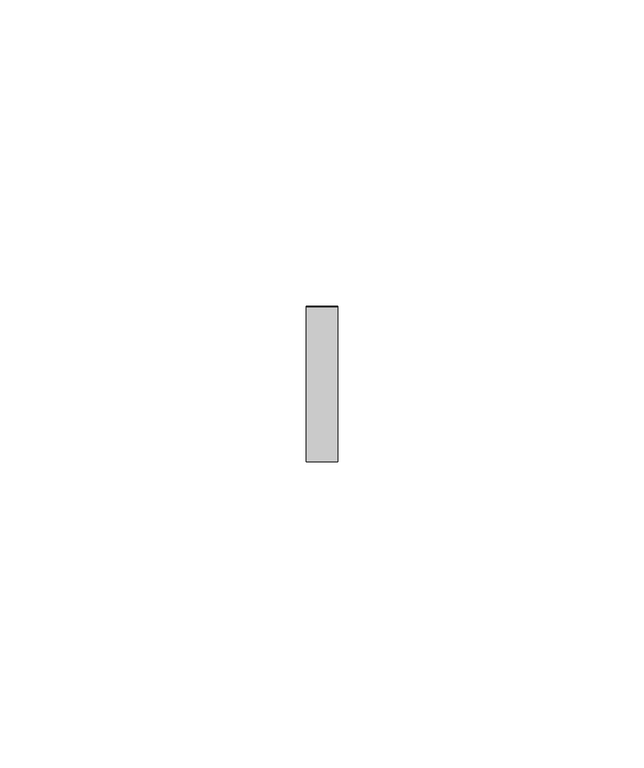
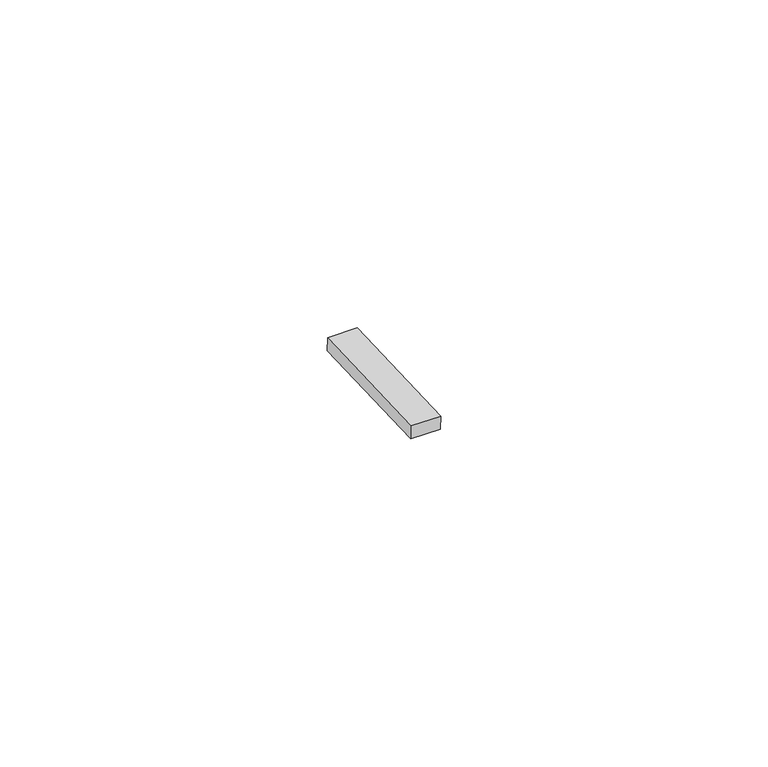
"""IFC4 building model written with IfcOpenShell, lengths in millimetres: proxy geometry, Inner panel:Inner panel:1:Inner panel:1 : Inner panel:Inner panel:300324:2:Inner panel:1:Inner panel:1 : Inner panel:Inner panel:300324:2 : Inner panel:Inner panel:1:Inner panel:1 : Inner panel:Inner panel:300324:300043:107 : Inner panel:Inner panel:1:Inner panel:1 : Inner panel:Inner panel:300324:2:Inner panel:1:Inner panel:1 : Inner panel:Inner panel:300324:2 : Inner panel:Inner panel:1:Inner panel:1 : Inner panel:Inner panel:300324:300043:308120."""

from ifc_helpers import new_model, si_unit, frame, origin, place, context, project, spatial, polyline, outline, extrude, source, transform, mapped, element, save


def generic_models_22f333e8(model_context):
    return source(origin(), model_context, "Body", "SweptSolid", [
        extrude(outline(polyline([(0.0, -25.3999999), (0.0, 0.0), (5.2138089, 0.0), (5.2138089, -25.3999999), (0.0, -25.3999999)])), frame((593530.195117, -577413.7950993, 4016.01903), z_axis=(0.0, -0.041630544712223896, 0.9991330730923502), x_axis=(-1.0, 0.0, 0.0)), (0.0, 0.0, 1.0), 2.4763745),
    ])


if __name__ == "__main__":
    model = new_model("IFC4")
    model_context = context("Model", 3, world=origin())
    ifc_project = project(units=[si_unit("LENGTHUNIT", "METRE", prefix="MILLI")], contexts=[model_context])
    site = spatial("IfcSite", under=ifc_project)
    building = spatial("IfcBuilding", under=site)
    placement = place(None, origin())
    generic_models_shape = generic_models_22f333e8(model_context)
    element("IfcBuildingElementProxy", 1, Name="Inner panel:Inner panel:1:Inner panel:1 : Inner panel:Inner panel:300324:2:Inner panel:1:Inner panel:1 : Inner panel:Inner panel:300324:2 : Inner panel:Inner panel:1:Inner panel:1 : Inner panel:Inner panel:300324:300043:107 : Inner panel:Inner panel:1:Inner panel:1 : Inner panel:Inner panel:300324:2:Inner panel:1:Inner panel:1 : Inner panel:Inner panel:300324:2 : Inner panel:Inner panel:1:Inner panel:1 : Inner panel:Inner panel:300324:300043:308120", ObjectType="Inner panel:Inner panel:1:Inner panel:1 : Inner panel:Inner panel:300324:2:Inner panel:1:Inner panel:1 : Inner panel:Inner panel:300324:2 : Inner panel:Inner panel:1:Inner panel:1 : Inner panel:Inner panel:300324:300043:107 : Inner panel:Inner panel:1:Inner panel:1 : Inner panel:Inner panel:300324:2:Inner panel:1:Inner panel:1 : Inner panel:Inner panel:300324:2 : Inner panel:Inner panel:1:Inner panel:1 : Inner panel:Inner panel:300324:300043:308120", at=placement, inside=building, context=model_context, shape_type="MappedRepresentation", body=[
        mapped(generic_models_shape, transform((0.0, 0.0, 0.0), x_axis=(1.0, 0.0, 0.0), y_axis=(0.0, 1.0, 0.0), z_axis=(0.0, 0.0, 1.0))),
    ])
    save(model, "model.ifc")

# Revit data of these elements
# Type "Inner panel:Inner panel:1:Inner panel:1 : Inner panel:Inner panel:300324:2:Inner panel:1:Inner panel:1 : Inner panel:Inner panel:300324:2 : Inner panel:Inner panel:1:Inner panel:1 : Inner panel:Inner panel:300324:300043:107 : Inner panel:Inner panel:1:Inner panel:1 : Inner panel:Inner panel:300324:2:Inner panel:1:Inner panel:1 : Inner panel:Inner panel:300324:2 : Inner panel:Inner panel:1:Inner panel:1 : Inner panel:Inner panel:300324:300043:308120"
#   NameOverride = "Inner panel:Inner panel:1:Inner panel:1 : Inner panel:Inner panel:300324:2:Inner panel:1:Inner panel:1 : Inner panel:Inner panel:300324:2 : Inner panel:Inner panel:1:Inner panel:1 : Inner panel:Inner panel:300324:300043:308120"
#   ObjectTypeOverride = "Inner panel:1:Inner panel:1 : Inner panel:Inner panel:300324:2 : Inner panel:Inner panel:1:Inner panel:1 : Inner panel:Inner panel:300324:300043"
#   Reference = "Inner panel"
#   Tag = "308120"
# Element 1 (IfcBuildingElementProxy, "Inner panel:Inner panel:1:Inner panel:1 : Inner panel:Inner panel:300324:2:Inner panel:1:Inner panel:1 : Inner panel:Inner panel:300324:2 : Inner panel:Inner panel:1:Inner panel:1 : Inner panel:Inner panel:300324:300043:107 : Inner panel:Inner panel:1:Inner panel:1 : Inner panel:Inner panel:300324:2:Inner panel:1:Inner panel:1 : Inner panel:Inner panel:300324:2 : Inner panel:Inner panel:1:Inner panel:1 : Inner panel:Inner panel:300324:300043:308120")
#   Materials on its faces: "AT CLIP - 1\" WIDE NON ABSORBENT, WEATHER-RESISTANT NEOPRENE/EPDM/SBR FOAM"
# Materials
#   "AT CLIP - 1\" WIDE NON ABSORBENT, WEATHER-RESISTANT NEOPRENE/EPDM/SBR FOAM": class "Generic", colour RGB 85 85 85, transparency 0, Cost = 0
